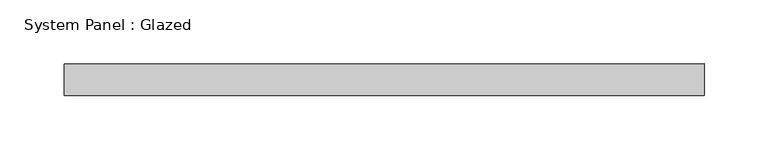
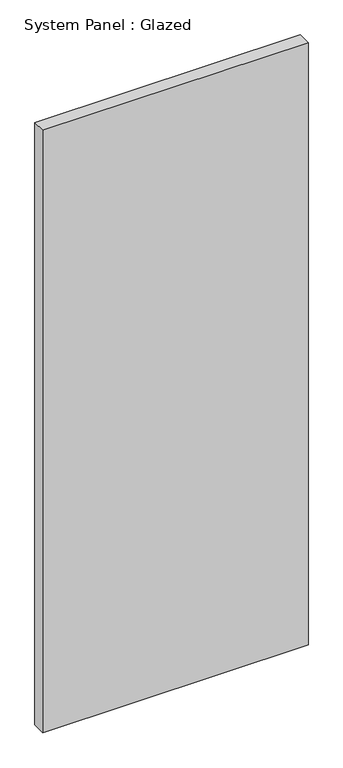
"""IFC4 building model written with IfcOpenShell, lengths in millimetres: plate geometry, System Panel : Glazed."""

from ifc_helpers import new_model, si_unit, origin, origin_with_axes, place, context, project, spatial, polyline, outline, extrude, source, transform, mapped, element, save


def system_panel_glazed_346501af(model_context):
    return source(origin(), model_context, "Body", "SweptSolid", [
        extrude(outline(polyline([(250.0, 24.5), (-250.0, 24.5), (-250.0, 49.5), (250.0, 49.5), (250.0, 24.5)])), origin_with_axes(), (0.0, 0.0, 1.0), 1200.0),
    ])


if __name__ == "__main__":
    model = new_model("IFC4")
    model_context = context("Model", 3, world=origin())
    ifc_project = project(units=[si_unit("LENGTHUNIT", "METRE", prefix="MILLI")], contexts=[model_context])
    site = spatial("IfcSite", under=ifc_project)
    building = spatial("IfcBuilding", under=site)
    placement = place(None, origin())
    system_panel_glazed_shape = system_panel_glazed_346501af(model_context)
    element("IfcPlate", 1, ObjectType="System Panel : Glazed", at=placement, inside=building, context=model_context, shape_type="MappedRepresentation", body=[
        mapped(system_panel_glazed_shape, transform((0.0, 0.0, 0.0), x_axis=(1.0, 0.0, 0.0), y_axis=(0.0, 1.0, 0.0), z_axis=(0.0, 0.0, 1.0))),
    ])
    save(model, "model.ifc")

# Revit data of these elements
# Element 1 (IfcPlate, "System Panel : Glazed")
#   Materials on its faces: "Glass"
# Materials
#   "Glass": class "Glass", colour RGB 218 227 224, transparency 0.85, Description = "Soda Lime Glass", Cost = 0
